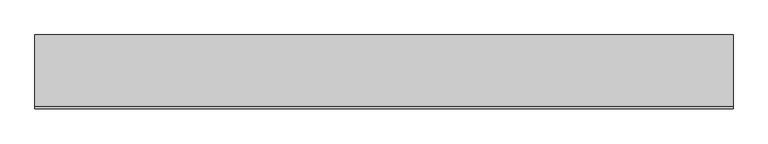
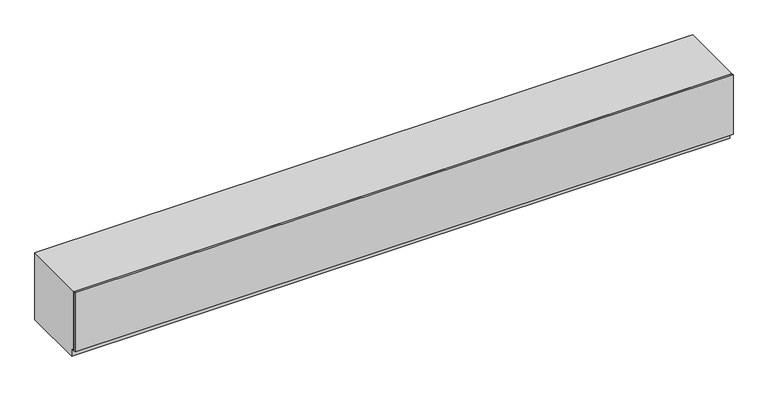
"""IFC4 building model written with IfcOpenShell, lengths in millimetres: furniture geometry, OD_CW_Base Cabinet : OD_CW_Base Cabinet."""

import ifcopenshell
import ifcopenshell.guid

model = None  # the IFC model being written
_history = None  # IfcOwnerHistory: only IFC2X3 demands one
_inside = {}  # id of a spatial element -> (the spatial element, [elements in it])
_under = {}  # id of a project, library or spatial element -> (it, [spatial elements below it])
_declared = {}  # id of a project -> (the project, [libraries it declares])
_typed = {}  # id of a type object -> (the type object, [elements of that type])
_made_of = {}  # id of a material, layer set ... -> (it, [elements and type objects made of it])


def new_model(schema):
    """Start an empty IFC model of exactly this schema.

    Asked for "IFC4X3", IfcOpenShell would pick the latest addendum, in which some entities
    have other attributes; the version numbers below select the first issue.
    IFC2X3 requires an IfcOwnerHistory on every rooted entity: one is made here for all.
    """
    global model, _history
    if schema == "IFC4X3":
        model = ifcopenshell.file(schema_version=(4, 3, 0, 0))
    else:
        model = ifcopenshell.file(schema=schema)
    _inside.clear()
    _under.clear()
    _declared.clear()
    _typed.clear()
    _made_of.clear()
    _history = None
    if model.schema == "IFC2X3":
        org = make("IfcOrganization", Name="unknown")
        user = make(
            "IfcPersonAndOrganization",
            ThePerson=make("IfcPerson", FamilyName="unknown"),
            TheOrganization=org,
        )
        app = make(
            "IfcApplication",
            ApplicationDeveloper=org,
            Version="unknown",
            ApplicationFullName="unknown",
            ApplicationIdentifier="unknown",
        )
        _history = make(
            "IfcOwnerHistory",
            OwningUser=user,
            OwningApplication=app,
            ChangeAction="ADDED",
            CreationDate=0,
        )
    return model


def make(cls, **values):
    """One entity of the class cls with the attributes given. An attribute that is None is left unset."""
    return model.create_entity(
        cls, **{name: value for name, value in values.items() if value is not None}
    )


def rooted(cls, **values):
    """An entity with a GlobalId (a new one), such as an element, a storey or a relation."""
    return make(cls, GlobalId=ifcopenshell.guid.new(), OwnerHistory=_history, **values)


def si_unit(unit_type, name, prefix=None):
    """IfcSIUnit, for example si_unit("LENGTHUNIT", "METRE", prefix="MILLI")."""
    return make("IfcSIUnit", UnitType=unit_type, Prefix=prefix, Name=name)


def assignment(units):
    """IfcUnitAssignment: the units of a project."""
    return None if units is None else make("IfcUnitAssignment", Units=units)


def point(xyz):
    """IfcCartesianPoint."""
    return None if xyz is None else make("IfcCartesianPoint", Coordinates=xyz)


def direction(xyz):
    """IfcDirection."""
    return None if xyz is None else make("IfcDirection", DirectionRatios=xyz)


def frame(location, z_axis=None, x_axis=None):
    """IfcAxis2Placement3D, a coordinate frame: its origin and axes. An axis left out is left unset."""
    return make(
        "IfcAxis2Placement3D",
        Location=point(location),
        Axis=direction(z_axis),
        RefDirection=direction(x_axis),
    )


def origin():
    """The frame at (0, 0, 0) with its axes left unset."""
    return frame((0.0, 0.0, 0.0))


def place(relative_to, where):
    """IfcLocalPlacement: puts the frame where relative to a parent placement (None: the world)."""
    return make(
        "IfcLocalPlacement", PlacementRelTo=relative_to, RelativePlacement=where
    )


def context(
    kind, dimensions, precision=None, world=None, true_north=None, identifier=None
):
    """IfcGeometricRepresentationContext, for example the 3D "Model" context."""
    return make(
        "IfcGeometricRepresentationContext",
        ContextIdentifier=identifier,
        ContextType=kind,
        CoordinateSpaceDimension=dimensions,
        Precision=precision,
        WorldCoordinateSystem=world,
        TrueNorth=true_north,
    )


def project(units=None, contexts=None):
    """IfcProject with its units and contexts."""
    return rooted(
        "IfcProject",
        Name="project",
        RepresentationContexts=contexts,
        UnitsInContext=assignment(units),
    )


def spatial(cls, under=None, at=None, **own):
    """A site, building, storey or space (cls), placed at a placement, below another one or the project."""
    s = rooted(cls, ObjectPlacement=at, **own)
    if under is not None:
        _under.setdefault(under.id(), (under, []))[1].append(s)
    return s


def polyline(points):
    """IfcPolyline through the points."""
    return make("IfcPolyline", Points=[point(p) for p in points])


def outline(outer, holes=None, kind="AREA"):
    """IfcArbitraryClosedProfileDef: a profile drawn as a closed curve; with holes, ...WithVoids."""
    if holes is None:
        return make("IfcArbitraryClosedProfileDef", ProfileType=kind, OuterCurve=outer)
    return make(
        "IfcArbitraryProfileDefWithVoids",
        ProfileType=kind,
        OuterCurve=outer,
        InnerCurves=holes,
    )


def extrude(swept, where, along, depth):
    """IfcExtrudedAreaSolid: the profile swept, set in the frame where, extruded along a direction by depth."""
    return make(
        "IfcExtrudedAreaSolid",
        SweptArea=swept,
        Position=where,
        ExtrudedDirection=direction(along),
        Depth=depth,
    )


def shape(context_of_items, identifier, shape_type, items):
    """IfcShapeRepresentation: the items that make up one representation, for example the "Body"."""
    return make(
        "IfcShapeRepresentation",
        ContextOfItems=context_of_items,
        RepresentationIdentifier=identifier,
        RepresentationType=shape_type,
        Items=items,
    )


def source(mapping_origin, context_of_items, identifier, shape_type, items):
    """IfcRepresentationMap: a shape defined once, which mapped items show again and again."""
    return make(
        "IfcRepresentationMap",
        MappingOrigin=mapping_origin,
        MappedRepresentation=shape(context_of_items, identifier, shape_type, items),
    )


def transform(
    local_origin,
    x_axis=None,
    y_axis=None,
    z_axis=None,
    scale=None,
    scale2=None,
    scale3=None,
    uniform=True,
):
    """IfcCartesianTransformationOperator3D, or its non-uniform kind. x_axis, y_axis, z_axis: its Axis1, 2, 3."""
    if uniform:
        return make(
            "IfcCartesianTransformationOperator3D",
            Axis1=direction(x_axis),
            Axis2=direction(y_axis),
            LocalOrigin=point(local_origin),
            Scale=scale,
            Axis3=direction(z_axis),
        )
    return make(
        "IfcCartesianTransformationOperator3DnonUniform",
        Axis1=direction(x_axis),
        Axis2=direction(y_axis),
        LocalOrigin=point(local_origin),
        Scale=scale,
        Axis3=direction(z_axis),
        Scale2=scale2,
        Scale3=scale3,
    )


def mapped(mapping_source, mapping_target):
    """IfcMappedItem: shows the shape of a source again, moved by a transform."""
    return make(
        "IfcMappedItem", MappingSource=mapping_source, MappingTarget=mapping_target
    )


def made_of(thing, what):
    """Note that an element or type object is made of a material, layer set ...; save() writes the relation."""
    if what is not None:
        _made_of.setdefault(what.id(), (what, []))[1].append(thing)
    return thing


def element(
    cls,
    number,
    at=None,
    inside=None,
    cuts=None,
    type_object=None,
    material=None,
    context=None,
    identifier="Body",
    shape_type=None,
    held_by="IfcProductDefinitionShape",
    body=None,
    shapes=None,
    **own,
):
    """One element of the class cls, such as IfcWall. Its Tag is "e" and its number.

    at: its placement. inside: the storey or other place that contains it. cuts: it is an
    opening in that element (IfcRelVoidsElement). A single representation is given by context,
    identifier, shape_type and body (its items); several are given by shapes. held_by: the class
    of the entity that holds the representations. save() writes the other relations.
    """
    e = rooted(cls, Tag="e%d" % number, ObjectPlacement=at, **own)
    if body is not None:
        shapes = [shape(context, identifier, shape_type, body)]
    if shapes is not None:
        e.Representation = make(held_by, Representations=shapes)
    if inside is not None:
        _inside.setdefault(inside.id(), (inside, []))[1].append(e)
    if cuts is not None:
        rooted(
            "IfcRelVoidsElement", RelatingBuildingElement=cuts, RelatedOpeningElement=e
        )
    if type_object is not None:
        _typed.setdefault(type_object.id(), (type_object, []))[1].append(e)
    return made_of(e, material)


def aggregate(whole, parts):
    """IfcRelAggregates: a whole, such as a stair, and the parts it consists of."""
    return rooted("IfcRelAggregates", RelatingObject=whole, RelatedObjects=parts)


def save(model, path):
    """Write the relations noted so far, then the file.

    IfcRelAggregates (storeys below a building ...), IfcRelContainedInSpatialStructure (elements
    in a storey), IfcRelDefinesByType, IfcRelAssociatesMaterial and IfcRelDeclares: one each for
    every whole, place, type object, material and project.
    """
    for whole, parts in _under.values():
        aggregate(whole, parts)
    for where, things in _inside.values():
        rooted(
            "IfcRelContainedInSpatialStructure",
            RelatedElements=things,
            RelatingStructure=where,
        )
    for kind, things in _typed.values():
        rooted("IfcRelDefinesByType", RelatedObjects=things, RelatingType=kind)
    for what, things in _made_of.values():
        rooted("IfcRelAssociatesMaterial", RelatedObjects=things, RelatingMaterial=what)
    for by, libraries in _declared.values():
        rooted("IfcRelDeclares", RelatingContext=by, RelatedDefinitions=libraries)
    model.write(path)


def furniture_2298d4ce(model_context):
    return source(origin(), model_context, "Body", "SweptSolid", [
        extrude(outline(polyline([(18.7377049, -228.6), (8167.5056128, -228.6), (8167.5056128, -254.0), (18.7377049, -254.0), (18.7377049, -228.6)])), frame((0.0, 0.0, 101.6), z_axis=(0.0, 0.0, 1.0), x_axis=(1.0, 0.0, 0.0)), (0.0, 0.0, 1.0), 774.7),
        extrude(outline(polyline([(-228.6, 876.3), (609.6, 876.3), (609.6, 0.0), (-177.8, 0.0), (-177.8, 101.6), (-228.6, 101.6), (-228.6, 876.3)])), frame((18.7377049, 0.0, 0.0), z_axis=(1.0, 0.0, 0.0), x_axis=(0.0, 1.0, 0.0)), (0.0, 0.0, 1.0), 8148.7679079),
    ])


if __name__ == "__main__":
    model = new_model("IFC4")
    model_context = context("Model", 3, world=origin())
    ifc_project = project(units=[si_unit("LENGTHUNIT", "METRE", prefix="MILLI")], contexts=[model_context])
    site = spatial("IfcSite", under=ifc_project)
    building = spatial("IfcBuilding", under=site)
    placement = place(None, origin())
    furniture_shape = furniture_2298d4ce(model_context)
    element("IfcFurniture", 1, ObjectType="OD_CW_Base Cabinet : OD_CW_Base Cabinet", at=placement, inside=building, context=model_context, shape_type="MappedRepresentation", body=[
        mapped(furniture_shape, transform((0.0, 0.0, 0.0), x_axis=(1.0, 0.0, 0.0), y_axis=(0.0, 1.0, 0.0), z_axis=(0.0, 0.0, 1.0))),
    ])
    save(model, "model.ifc")

# Revit data of these elements
# Type "OD_CW_Base Cabinet : OD_CW_Base Cabinet"
#   OD_CW_Width [instance default] = 2' - 10"
#   OD_CW_Length [instance default] = 8' - 0"
#   OD_CW_Height [instance default] = 2' - 3"
#   Depth = 2' - 0"
#   Height = 3' - 0"
#   Width = 4' - 0"
#   OD_CW_Material_Front Panel [instance default] = none
#   OD_CW_Material_Body [instance default] = none
# Element 1 (IfcFurniture, "OD_CW_Base Cabinet : OD_CW_Base Cabinet")
#   OD_CW_Length = 26' - 8.81763"
#   OD_CW_Height = 2' - 10 1/2"
#   OD_CW_Material_Front Panel = WOOD-OAKFIRE
#   OD_CW_Material_Body = WOOD-OAKFIRE
#   Materials on its faces: "WOOD-OAKFIRE"
# Materials
#   "WOOD-OAKFIRE": class "Wood", colour RGB 198 202 183, transparency 0, Description = "Generic wood", Cost = 0
